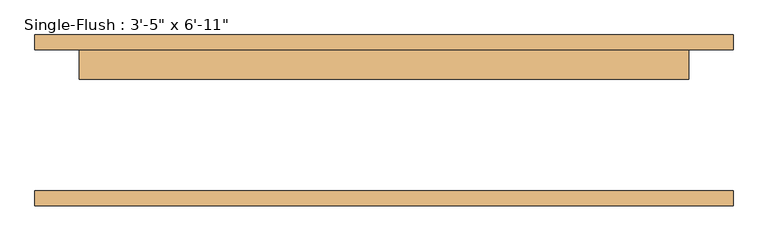
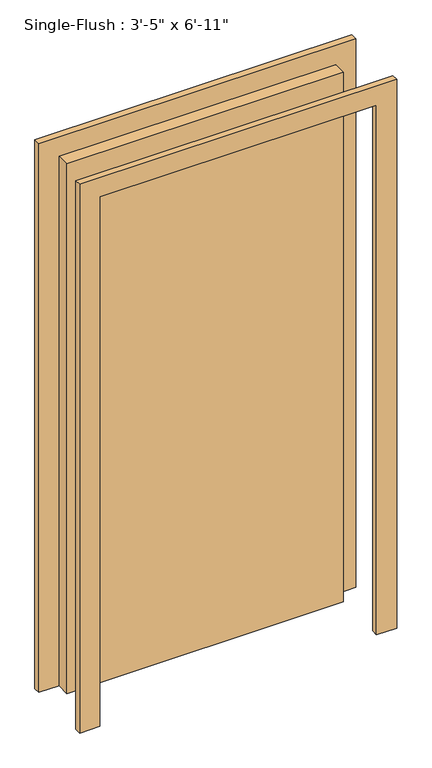
"""IFC4 building model written with IfcOpenShell, lengths in millimetres: door geometry."""

from ifc_helpers import new_model, si_unit, frame, origin, origin_with_axes, place, context, project, spatial, polyline, outline, extrude, source, transform, mapped, element, save


def door_eaa92909(model_context):
    return source(origin(), model_context, "Body", "SweptSolid", [
        extrude(outline(polyline([(2184.4, -596.9), (0.0, -596.9), (0.0, -520.7), (2108.2, -520.7), (2108.2, 520.7), (0.0, 520.7), (0.0, 596.9), (2184.4, 596.9), (2184.4, -596.9)])), frame((0.0, 120.65, 0.0), z_axis=(0.0, 1.0, 0.0), x_axis=(0.0, 0.0, 1.0)), (0.0, 0.0, 1.0), 25.4),
        extrude(outline(polyline([(2184.4, 596.9), (2184.4, -596.9), (0.0, -596.9), (0.0, -520.7), (2108.2, -520.7), (2108.2, 520.7), (0.0, 520.7), (0.0, 596.9), (2184.4, 596.9)])), frame((0.0, -146.05, 0.0), z_axis=(0.0, 1.0, 0.0), x_axis=(0.0, 0.0, 1.0)), (0.0, 0.0, 1.0), 25.4),
        extrude(outline(polyline([(520.7, 69.85), (-520.7, 69.85), (-520.7, 120.65), (520.7, 120.65), (520.7, 69.85)])), origin_with_axes(), (0.0, 0.0, 1.0), 2108.2),
    ])


if __name__ == "__main__":
    model = new_model("IFC4")
    model_context = context("Model", 3, world=origin())
    ifc_project = project(units=[si_unit("LENGTHUNIT", "METRE", prefix="MILLI")], contexts=[model_context])
    site = spatial("IfcSite", under=ifc_project)
    building = spatial("IfcBuilding", under=site)
    placement = place(None, origin())
    door_shape = door_eaa92909(model_context)
    element("IfcDoor", 1, ObjectType="Single-Flush : 3'-5\" x 6'-11\"", at=placement, inside=building, context=model_context, shape_type="MappedRepresentation", body=[
        mapped(door_shape, transform((0.0, 0.0, 0.0), x_axis=(1.0, 0.0, 0.0), y_axis=(0.0, 1.0, 0.0), z_axis=(0.0, 0.0, 1.0))),
    ])
    save(model, "model.ifc")

# Revit data of these elements
# Type "Single-Flush : 3'-5\" x 6'-11\""
#   Type Mark = "9"
#   Construction Type Id = "MDOOR"
#   Assembly Code = "C1020"
#   Analytic Construction = "Metal"
#   Thickness = 0' - 2"
#   Heat Transfer Coefficient (U) = 3.7021 W/(m²·K)
#   Height = 6' - 11"
#   Trim Projection Ext = 0' - 1"
#   Trim Projection Int = 0' - 1"
#   Trim Width = 0' - 3"
#   Width = 3' - 5"
#   Door Material = Door - Panel
#   Frame Material = Door - Frame
#   Visual Light Transmittance = 0
#   Solar Heat Gain Coefficient = 0
#   Function = (empty or 0)
#   Wall Closure = (empty or 0)
# Element 1 (IfcDoor, "Single-Flush : 3'-5\" x 6'-11\"")
#   Materials on its faces: "Door - Frame", "Door - Panel"
# Materials
#   "Door - Panel": class "Wood", colour RGB 210 159 95, transparency 0, Cost = 0
#   "Door - Frame": class "Miscellaneous", colour RGB 118 70 51, transparency 0, Cost = 0
